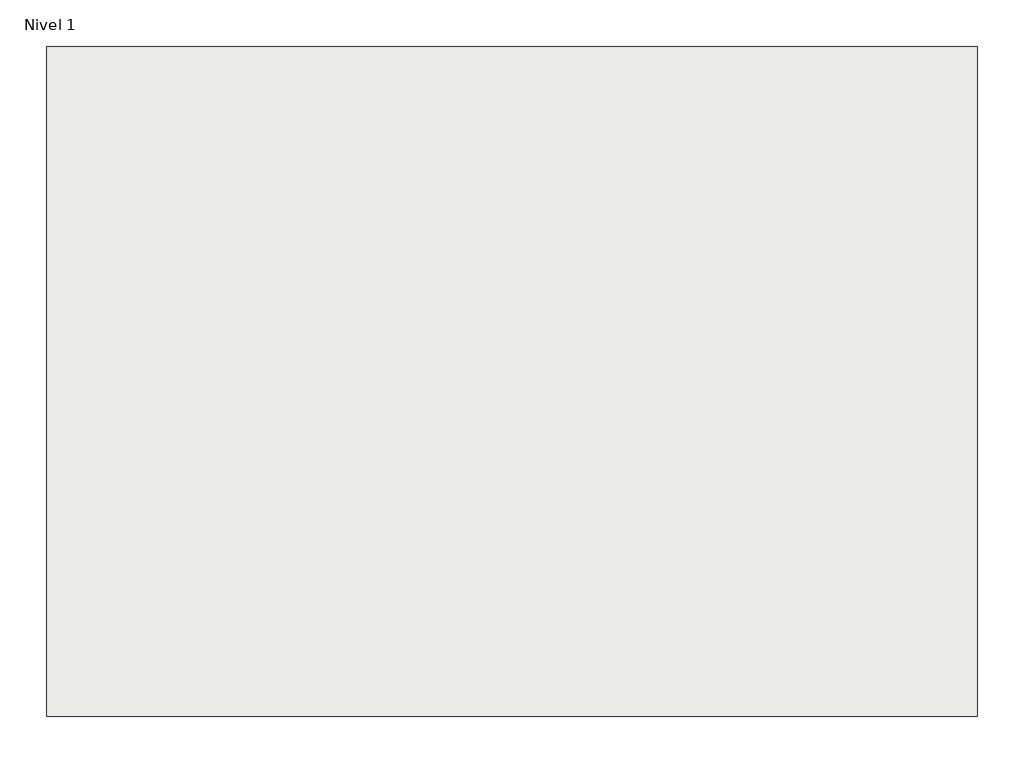
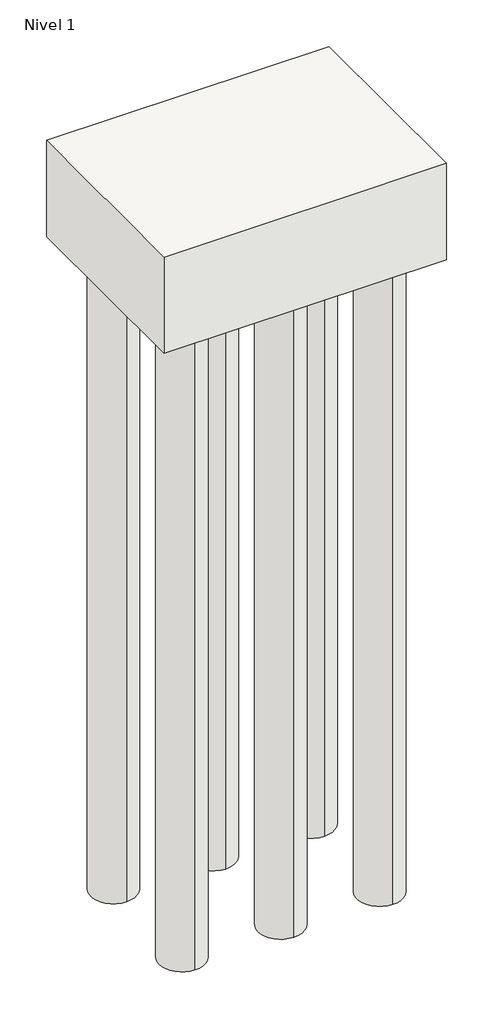
# One storey: 7 slabs.
"""IFC4 building model written with IfcOpenShell, lengths in millimetres."""

from ifc_helpers import new_model, si_unit, point, frame, frame_2d, origin, place, context, project, spatial, polyline, circle_curve, trimmed, segment, composite_curve, outline, extrude, element, save

model = new_model("IFC4")

# Units and contexts
model_context = context("Model", 3, world=origin())
ifc_project = project(units=[si_unit("LENGTHUNIT", "METRE", prefix="MILLI")], contexts=[model_context])

# Site, building, storey
site = spatial("IfcSite", under=ifc_project)
building = spatial("IfcBuilding", under=site)
storey = spatial("IfcBuildingStorey", under=building, Name="Nivel 1", Elevation=0.0)

# Slabs
placement = place(None, origin())
element("IfcSlab", 1, ObjectType="M_Pilote-Tubería de acero : Diámetro 400 mm", at=placement, inside=storey, context=model_context, shape_type="SweptSolid", body=[
    extrude(outline(composite_curve([segment(trimmed(circle_curve(frame_2d((2647.9922387, -176.7292509)), 200.0), [point((2647.9922387, -376.7292509))], [point((2647.9922387, 23.2707491))], False, "CARTESIAN"), True, "CONTINUOUS"), segment(trimmed(circle_curve(frame_2d((2647.9922387, -176.7292509)), 200.0), [point((2647.9922387, 23.2707491))], [point((2647.9922387, -376.7292509))], False, "CARTESIAN"), True, "CONTINUOUS")], self_intersect=False)), frame((0.0, 0.0, -6900.0), z_axis=(0.0, 0.0, 1.0), x_axis=(1.0, 0.0, 0.0)), (0.0, 0.0, 1.0), 6000.0),
])
element("IfcSlab", 2, ObjectType="M_Pilote-Tubería de acero : Diámetro 400 mm", at=placement, inside=storey, context=model_context, shape_type="SweptSolid", body=[
    extrude(outline(composite_curve([segment(trimmed(circle_curve(frame_2d((2647.9922387, 873.2707491)), 200.0), [point((2647.9922387, 673.2707491))], [point((2647.9922387, 1073.2707491))], False, "CARTESIAN"), True, "CONTINUOUS"), segment(trimmed(circle_curve(frame_2d((2647.9922387, 873.2707491)), 200.0), [point((2647.9922387, 1073.2707491))], [point((2647.9922387, 673.2707491))], False, "CARTESIAN"), True, "CONTINUOUS")], self_intersect=False)), frame((0.0, 0.0, -6900.0), z_axis=(0.0, 0.0, 1.0), x_axis=(1.0, 0.0, 0.0)), (0.0, 0.0, 1.0), 6000.0),
])
element("IfcSlab", 3, ObjectType="M_Pilote-Tubería de acero : Diámetro 400 mm", at=placement, inside=storey, context=model_context, shape_type="SweptSolid", body=[
    extrude(outline(composite_curve([segment(trimmed(circle_curve(frame_2d((897.9922387, 873.2707491)), 200.0), [point((897.9922387, 673.2707491))], [point((897.9922387, 1073.2707491))], False, "CARTESIAN"), True, "CONTINUOUS"), segment(trimmed(circle_curve(frame_2d((897.9922387, 873.2707491)), 200.0), [point((897.9922387, 1073.2707491))], [point((897.9922387, 673.2707491))], False, "CARTESIAN"), True, "CONTINUOUS")], self_intersect=False)), frame((0.0, 0.0, -6900.0), z_axis=(0.0, 0.0, 1.0), x_axis=(1.0, 0.0, 0.0)), (0.0, 0.0, 1.0), 6000.0),
])
element("IfcSlab", 4, ObjectType="M_Pilote-Tubería de acero : Diámetro 400 mm", at=placement, inside=storey, context=model_context, shape_type="SweptSolid", body=[
    extrude(outline(composite_curve([segment(trimmed(circle_curve(frame_2d((897.9922387, -176.7292509)), 200.0), [point((897.9922387, -376.7292509))], [point((897.9922387, 23.2707491))], False, "CARTESIAN"), True, "CONTINUOUS"), segment(trimmed(circle_curve(frame_2d((897.9922387, -176.7292509)), 200.0), [point((897.9922387, 23.2707491))], [point((897.9922387, -376.7292509))], False, "CARTESIAN"), True, "CONTINUOUS")], self_intersect=False)), frame((0.0, 0.0, -6900.0), z_axis=(0.0, 0.0, 1.0), x_axis=(1.0, 0.0, 0.0)), (0.0, 0.0, 1.0), 6000.0),
])
element("IfcSlab", 5, ObjectType="M_Pilote-Tubería de acero : Diámetro 400 mm", at=placement, inside=storey, context=model_context, shape_type="SweptSolid", body=[
    extrude(outline(composite_curve([segment(trimmed(circle_curve(frame_2d((1772.9922387, -176.7292509)), 200.0), [point((1772.9922387, -376.7292509))], [point((1772.9922387, 23.2707491))], False, "CARTESIAN"), True, "CONTINUOUS"), segment(trimmed(circle_curve(frame_2d((1772.9922387, -176.7292509)), 200.0), [point((1772.9922387, 23.2707491))], [point((1772.9922387, -376.7292509))], False, "CARTESIAN"), True, "CONTINUOUS")], self_intersect=False)), frame((0.0, 0.0, -6900.0), z_axis=(0.0, 0.0, 1.0), x_axis=(1.0, 0.0, 0.0)), (0.0, 0.0, 1.0), 6000.0),
])
element("IfcSlab", 6, ObjectType="M_Pilote-Tubería de acero : Diámetro 400 mm", at=placement, inside=storey, context=model_context, shape_type="SweptSolid", body=[
    extrude(outline(composite_curve([segment(trimmed(circle_curve(frame_2d((1772.9922387, 873.2707491)), 200.0), [point((1772.9922387, 673.2707491))], [point((1772.9922387, 1073.2707491))], False, "CARTESIAN"), True, "CONTINUOUS"), segment(trimmed(circle_curve(frame_2d((1772.9922387, 873.2707491)), 200.0), [point((1772.9922387, 1073.2707491))], [point((1772.9922387, 673.2707491))], False, "CARTESIAN"), True, "CONTINUOUS")], self_intersect=False)), frame((0.0, 0.0, -6900.0), z_axis=(0.0, 0.0, 1.0), x_axis=(1.0, 0.0, 0.0)), (0.0, 0.0, 1.0), 6000.0),
])
element("IfcSlab", 7, ObjectType="Remate de pilote-6 pilotes : 2500 x 1800 x 900mm", at=placement, inside=storey, context=model_context, shape_type="SweptSolid", body=[
    extrude(outline(polyline([(522.9922387, 1248.2707491), (3022.9922387, 1248.2707491), (3022.9922387, -551.7292509), (522.9922387, -551.7292509), (522.9922387, 1248.2707491)])), frame((0.0, 0.0, -900.0), z_axis=(0.0, 0.0, 1.0), x_axis=(1.0, 0.0, 0.0)), (0.0, 0.0, 1.0), 900.0),
])

save(model, "model.ifc")

# Revit data of these elements
# Project information
#   Fecha de emisión de proyecto = "Fecha de emisión"
#   Estado de proyecto = "Estado de proyecto"
#   Nombre de cliente = "Propietario"
#   Dirección de proyecto = "Introduzca dirección aquí"
#   Nombre de proyecto = "Nombre de proyecto"
#   Número de proyecto = "0001"
# Type "M_Pilote-Tubería de acero : Diámetro 400 mm"
#   Assembly Code = "A1020130"
#   Radio = 0.200 m
#   Incrustación mínima = 0.150 m
#   Diameter = 0.400 m
#   Depth = 6.000 m
#   Structural Material [instance default] = Metal - Acero - 345 MPa
# Type "Remate de pilote-6 pilotes : 2500 x 1800 x 900mm"
#   Assembly Code = "A1010130"
#   Width = 1.800 m
#   Thickness = 0.900 m
#   Length = 2.500 m
#   Límite = 0.150 m
#   Espacio libre = 0.375 m
#   Structural Material [instance default] = Hormigón - Hormigón moldeado in situ
#   Tipo de pilote = M_Pilote-Tubería de acero : Diámetro 400 mm
# Elements 1, 2, 3, 4, 5, 6 (IfcSlab, "M_Pilote-Tubería de acero : Diámetro 400 mm")
#   Structural Material = Metal - Acero - 345 MPa
#   Phase Created = Nueva construcción
#   Materials on its faces: "Metal - Acero - 345 MPa"
# Element 7 (IfcSlab, "Remate de pilote-6 pilotes : 2500 x 1800 x 900mm")
#   Structural Material = Hormigón - Hormigón moldeado in situ
#   Phase Created = Nueva construcción
#   Materials on its faces: "Hormigón - Hormigón moldeado in situ"
# Materials
#   "Metal - Acero - 345 MPa": class "Metal", colour RGB 247 247 247, transparency 0
#   "Hormigón - Hormigón moldeado in situ": class "Hormigón", colour RGB 192 192 192, transparency 0
